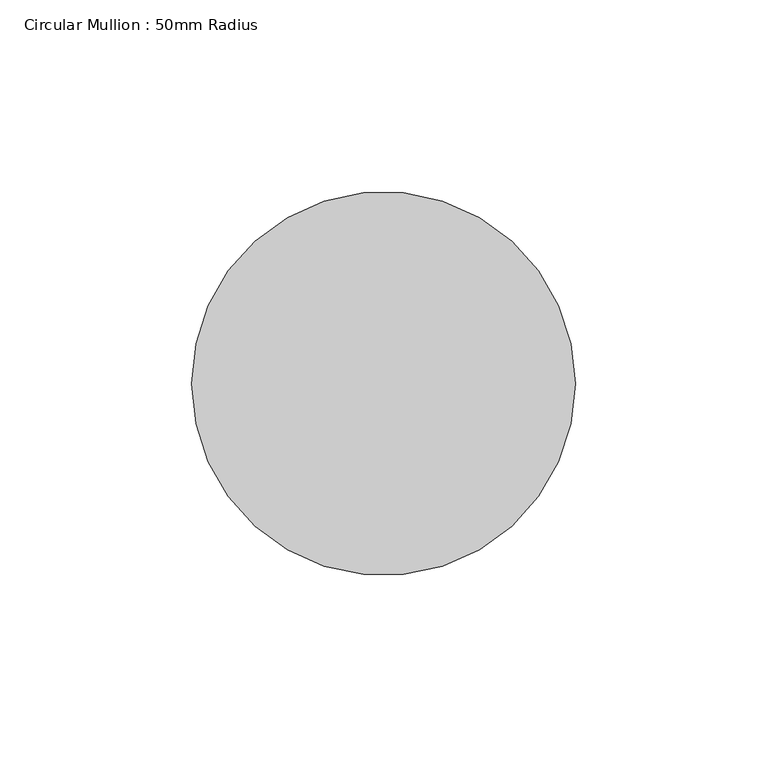
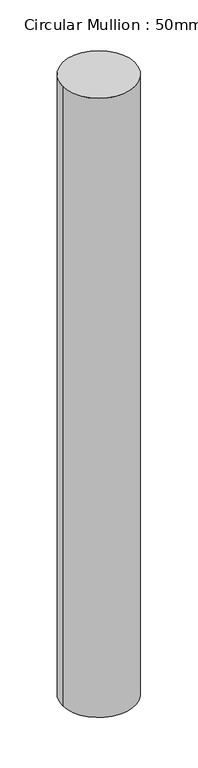
"""IFC4 building model written with IfcOpenShell, lengths in millimetres: member geometry, Circular Mullion : 50mm Radius."""

from ifc_helpers import new_model, si_unit, point, frame, origin, origin_2d, place, context, project, spatial, circle_curve, trimmed, segment, composite_curve, outline, extrude, source, transform, mapped, element, save


def circular_mullion_50mm_radius_7f89396d(model_context):
    return source(origin(), model_context, "Body", "SweptSolid", [
        extrude(outline(composite_curve([segment(trimmed(circle_curve(origin_2d(), 50.0), [point((50.0, 0.0))], [point((-50.0, 0.0))], False, "CARTESIAN"), True, "CONTINUOUS"), segment(trimmed(circle_curve(origin_2d(), 50.0), [point((-50.0, 0.0))], [point((50.0, 0.0))], False, "CARTESIAN"), True, "CONTINUOUS")], self_intersect=False)), frame((0.0, 0.0, -905.192682), z_axis=(0.0, 0.0, 1.0), x_axis=(1.0, 0.0, 0.0)), (0.0, 0.0, 1.0), 905.192682),
    ])


if __name__ == "__main__":
    model = new_model("IFC4")
    model_context = context("Model", 3, world=origin())
    ifc_project = project(units=[si_unit("LENGTHUNIT", "METRE", prefix="MILLI")], contexts=[model_context])
    site = spatial("IfcSite", under=ifc_project)
    building = spatial("IfcBuilding", under=site)
    placement = place(None, origin())
    circular_mullion_50mm_radius_shape = circular_mullion_50mm_radius_7f89396d(model_context)
    element("IfcMember", 1, ObjectType="Circular Mullion : 50mm Radius", at=placement, inside=building, context=model_context, shape_type="MappedRepresentation", body=[
        mapped(circular_mullion_50mm_radius_shape, transform((0.0, 0.0, 0.0), x_axis=(1.0, 0.0, 0.0), y_axis=(0.0, 1.0, 0.0), z_axis=(0.0, 0.0, 1.0))),
    ])
    save(model, "model.ifc")

# Revit data of these elements
# Type "Circular Mullion : 50mm Radius"
#   built-in parameter 1007350 = 0.164042 (stored number, unit not read)
# Element 1 (IfcMember, "Circular Mullion : 50mm Radius")
#   Materials on its faces: "Aluminium"
# Materials
#   "Aluminium": class "Metal", colour RGB 247 247 247, transparency 0, Description = "Aluminium 6061", Cost = 0
